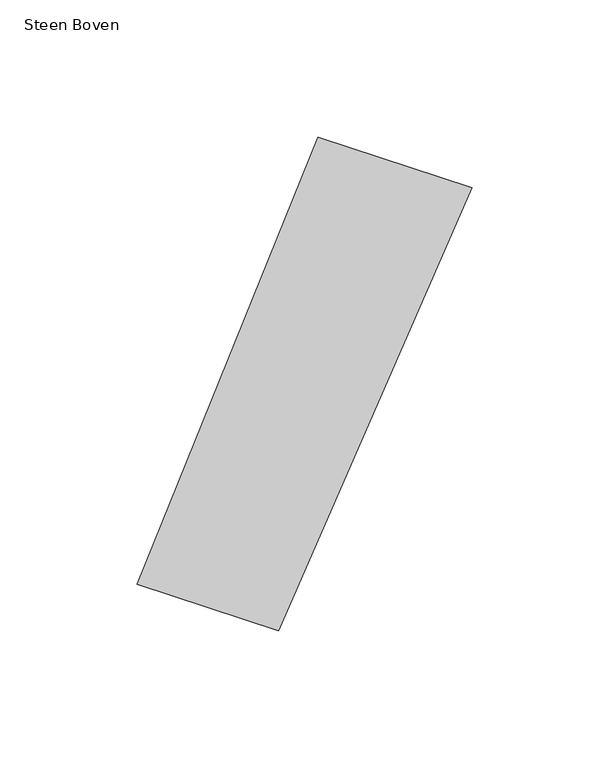
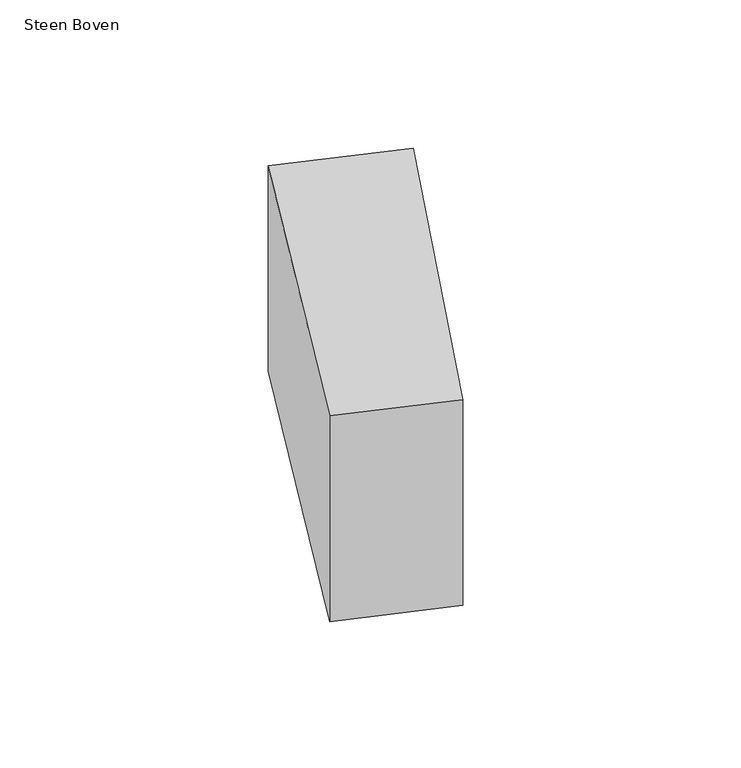
"""IFC4 building model written with IfcOpenShell, lengths in millimetres: proxy geometry, 00_GMA_steen_versie_4 : Steen Boven."""

from ifc_helpers import new_model, si_unit, origin, origin_with_axes, place, context, project, spatial, polyline, outline, extrude, source, transform, mapped, element, save


def steen_boven_d1918d28(model_context):
    return source(origin(), model_context, "Body", "SweptSolid", [
        extrude(outline(polyline([(136.9542889, 153.0212994), (66.6439439, -8.1457475), (15.1759982, 8.6415327), (80.8921587, 171.2961397), (136.9542889, 153.0212994)])), origin_with_axes(), (0.0, 0.0, 1.0), 100.0),
    ])


if __name__ == "__main__":
    model = new_model("IFC4")
    model_context = context("Model", 3, world=origin())
    ifc_project = project(units=[si_unit("LENGTHUNIT", "METRE", prefix="MILLI")], contexts=[model_context])
    site = spatial("IfcSite", under=ifc_project)
    building = spatial("IfcBuilding", under=site)
    placement = place(None, origin())
    steen_boven_shape = steen_boven_d1918d28(model_context)
    element("IfcBuildingElementProxy", 1, Name="00_GMA_steen_versie_4 : Steen Boven", ObjectType="00_GMA_steen_versie_4 : Steen Boven", at=placement, inside=building, context=model_context, shape_type="MappedRepresentation", body=[
        mapped(steen_boven_shape, transform((0.0, 0.0, 0.0), x_axis=(1.0, 0.0, 0.0), y_axis=(0.0, 1.0, 0.0), z_axis=(0.0, 0.0, 1.0))),
    ])
    save(model, "model.ifc")

# Revit data of these elements
# Type "00_GMA_steen_versie_4 : Steen Boven"
#   StootVoegHalfBoven [instance default] = 5 mm
#   StootVoegHalf [instance default] = 5 mm
#   StootVoegBreedteOnder = 10 mm
#   StootVoegBreedteBoven = 10 mm
#   Steendikte = 100 mm
#   LintVoegOnderHalf = 5 mm
#   LintVoegOnder = 10 mm
#   LintVoegBovenHalf = 0 mm
#   LintVoegBoven = 0 mm
#   materiaal = none
#   MateriaalVoeg = none
#   Default Elevation = 0
